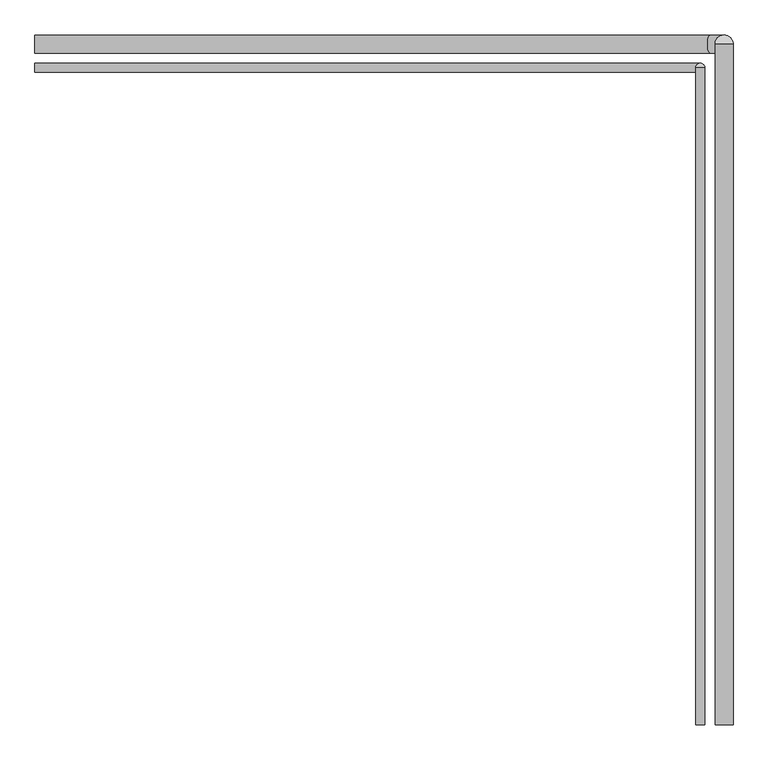
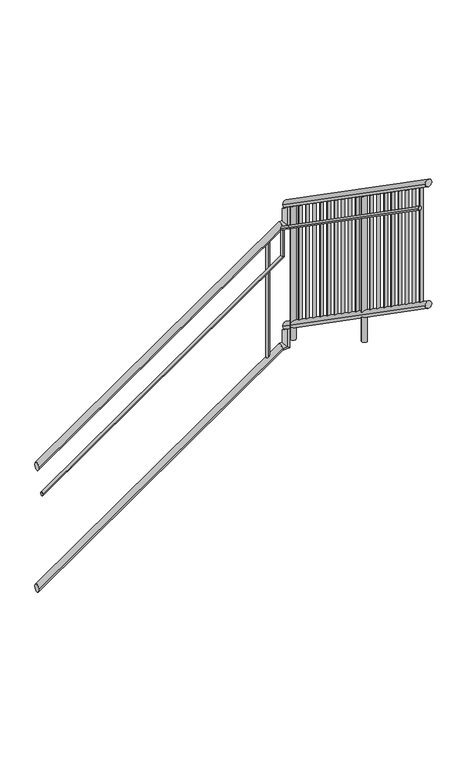
"""IFC4 building model written with IfcOpenShell, lengths in millimetres: railing geometry."""

import ifcopenshell
import ifcopenshell.guid

model = None  # the IFC model being written
_history = None  # IfcOwnerHistory: only IFC2X3 demands one
_inside = {}  # id of a spatial element -> (the spatial element, [elements in it])
_under = {}  # id of a project, library or spatial element -> (it, [spatial elements below it])
_declared = {}  # id of a project -> (the project, [libraries it declares])
_typed = {}  # id of a type object -> (the type object, [elements of that type])
_made_of = {}  # id of a material, layer set ... -> (it, [elements and type objects made of it])


def new_model(schema):
    """Start an empty IFC model of exactly this schema.

    Asked for "IFC4X3", IfcOpenShell would pick the latest addendum, in which some entities
    have other attributes; the version numbers below select the first issue.
    IFC2X3 requires an IfcOwnerHistory on every rooted entity: one is made here for all.
    """
    global model, _history
    if schema == "IFC4X3":
        model = ifcopenshell.file(schema_version=(4, 3, 0, 0))
    else:
        model = ifcopenshell.file(schema=schema)
    _inside.clear()
    _under.clear()
    _declared.clear()
    _typed.clear()
    _made_of.clear()
    _history = None
    if model.schema == "IFC2X3":
        org = make("IfcOrganization", Name="unknown")
        user = make(
            "IfcPersonAndOrganization",
            ThePerson=make("IfcPerson", FamilyName="unknown"),
            TheOrganization=org,
        )
        app = make(
            "IfcApplication",
            ApplicationDeveloper=org,
            Version="unknown",
            ApplicationFullName="unknown",
            ApplicationIdentifier="unknown",
        )
        _history = make(
            "IfcOwnerHistory",
            OwningUser=user,
            OwningApplication=app,
            ChangeAction="ADDED",
            CreationDate=0,
        )
    return model


def make(cls, **values):
    """One entity of the class cls with the attributes given. An attribute that is None is left unset."""
    return model.create_entity(
        cls, **{name: value for name, value in values.items() if value is not None}
    )


def rooted(cls, **values):
    """An entity with a GlobalId (a new one), such as an element, a storey or a relation."""
    return make(cls, GlobalId=ifcopenshell.guid.new(), OwnerHistory=_history, **values)


def si_unit(unit_type, name, prefix=None):
    """IfcSIUnit, for example si_unit("LENGTHUNIT", "METRE", prefix="MILLI")."""
    return make("IfcSIUnit", UnitType=unit_type, Prefix=prefix, Name=name)


def assignment(units):
    """IfcUnitAssignment: the units of a project."""
    return None if units is None else make("IfcUnitAssignment", Units=units)


def point(xyz):
    """IfcCartesianPoint."""
    return None if xyz is None else make("IfcCartesianPoint", Coordinates=xyz)


def direction(xyz):
    """IfcDirection."""
    return None if xyz is None else make("IfcDirection", DirectionRatios=xyz)


def frame(location, z_axis=None, x_axis=None):
    """IfcAxis2Placement3D, a coordinate frame: its origin and axes. An axis left out is left unset."""
    return make(
        "IfcAxis2Placement3D",
        Location=point(location),
        Axis=direction(z_axis),
        RefDirection=direction(x_axis),
    )


def origin():
    """The frame at (0, 0, 0) with its axes left unset."""
    return frame((0.0, 0.0, 0.0))


def place(relative_to, where):
    """IfcLocalPlacement: puts the frame where relative to a parent placement (None: the world)."""
    return make(
        "IfcLocalPlacement", PlacementRelTo=relative_to, RelativePlacement=where
    )


def context(
    kind, dimensions, precision=None, world=None, true_north=None, identifier=None
):
    """IfcGeometricRepresentationContext, for example the 3D "Model" context."""
    return make(
        "IfcGeometricRepresentationContext",
        ContextIdentifier=identifier,
        ContextType=kind,
        CoordinateSpaceDimension=dimensions,
        Precision=precision,
        WorldCoordinateSystem=world,
        TrueNorth=true_north,
    )


def project(units=None, contexts=None):
    """IfcProject with its units and contexts."""
    return rooted(
        "IfcProject",
        Name="project",
        RepresentationContexts=contexts,
        UnitsInContext=assignment(units),
    )


def spatial(cls, under=None, at=None, **own):
    """A site, building, storey or space (cls), placed at a placement, below another one or the project."""
    s = rooted(cls, ObjectPlacement=at, **own)
    if under is not None:
        _under.setdefault(under.id(), (under, []))[1].append(s)
    return s


def circle_curve(where, radius):
    """IfcCircle in the frame where."""
    return make("IfcCircle", Position=where, Radius=radius)


def ellipse_curve(where, semi_axis1, semi_axis2):
    """IfcEllipse in the frame where."""
    return make(
        "IfcEllipse", Position=where, SemiAxis1=semi_axis1, SemiAxis2=semi_axis2
    )


def shape(context_of_items, identifier, shape_type, items):
    """IfcShapeRepresentation: the items that make up one representation, for example the "Body"."""
    return make(
        "IfcShapeRepresentation",
        ContextOfItems=context_of_items,
        RepresentationIdentifier=identifier,
        RepresentationType=shape_type,
        Items=items,
    )


def source(mapping_origin, context_of_items, identifier, shape_type, items):
    """IfcRepresentationMap: a shape defined once, which mapped items show again and again."""
    return make(
        "IfcRepresentationMap",
        MappingOrigin=mapping_origin,
        MappedRepresentation=shape(context_of_items, identifier, shape_type, items),
    )


def transform(
    local_origin,
    x_axis=None,
    y_axis=None,
    z_axis=None,
    scale=None,
    scale2=None,
    scale3=None,
    uniform=True,
):
    """IfcCartesianTransformationOperator3D, or its non-uniform kind. x_axis, y_axis, z_axis: its Axis1, 2, 3."""
    if uniform:
        return make(
            "IfcCartesianTransformationOperator3D",
            Axis1=direction(x_axis),
            Axis2=direction(y_axis),
            LocalOrigin=point(local_origin),
            Scale=scale,
            Axis3=direction(z_axis),
        )
    return make(
        "IfcCartesianTransformationOperator3DnonUniform",
        Axis1=direction(x_axis),
        Axis2=direction(y_axis),
        LocalOrigin=point(local_origin),
        Scale=scale,
        Axis3=direction(z_axis),
        Scale2=scale2,
        Scale3=scale3,
    )


def mapped(mapping_source, mapping_target):
    """IfcMappedItem: shows the shape of a source again, moved by a transform."""
    return make(
        "IfcMappedItem", MappingSource=mapping_source, MappingTarget=mapping_target
    )


def made_of(thing, what):
    """Note that an element or type object is made of a material, layer set ...; save() writes the relation."""
    if what is not None:
        _made_of.setdefault(what.id(), (what, []))[1].append(thing)
    return thing


def element(
    cls,
    number,
    at=None,
    inside=None,
    cuts=None,
    type_object=None,
    material=None,
    context=None,
    identifier="Body",
    shape_type=None,
    held_by="IfcProductDefinitionShape",
    body=None,
    shapes=None,
    **own,
):
    """One element of the class cls, such as IfcWall. Its Tag is "e" and its number.

    at: its placement. inside: the storey or other place that contains it. cuts: it is an
    opening in that element (IfcRelVoidsElement). A single representation is given by context,
    identifier, shape_type and body (its items); several are given by shapes. held_by: the class
    of the entity that holds the representations. save() writes the other relations.
    """
    e = rooted(cls, Tag="e%d" % number, ObjectPlacement=at, **own)
    if body is not None:
        shapes = [shape(context, identifier, shape_type, body)]
    if shapes is not None:
        e.Representation = make(held_by, Representations=shapes)
    if inside is not None:
        _inside.setdefault(inside.id(), (inside, []))[1].append(e)
    if cuts is not None:
        rooted(
            "IfcRelVoidsElement", RelatingBuildingElement=cuts, RelatedOpeningElement=e
        )
    if type_object is not None:
        _typed.setdefault(type_object.id(), (type_object, []))[1].append(e)
    return made_of(e, material)


def aggregate(whole, parts):
    """IfcRelAggregates: a whole, such as a stair, and the parts it consists of."""
    return rooted("IfcRelAggregates", RelatingObject=whole, RelatedObjects=parts)


def save(model, path):
    """Write the relations noted so far, then the file.

    IfcRelAggregates (storeys below a building ...), IfcRelContainedInSpatialStructure (elements
    in a storey), IfcRelDefinesByType, IfcRelAssociatesMaterial and IfcRelDeclares: one each for
    every whole, place, type object, material and project.
    """
    for whole, parts in _under.values():
        aggregate(whole, parts)
    for where, things in _inside.values():
        rooted(
            "IfcRelContainedInSpatialStructure",
            RelatedElements=things,
            RelatingStructure=where,
        )
    for kind, things in _typed.values():
        rooted("IfcRelDefinesByType", RelatedObjects=things, RelatingType=kind)
    for what, things in _made_of.values():
        rooted("IfcRelAssociatesMaterial", RelatedObjects=things, RelatingMaterial=what)
    for by, libraries in _declared.values():
        rooted("IfcRelDeclares", RelatingContext=by, RelatedDefinitions=libraries)
    model.write(path)


def plane_surface(at):
    """IfcPlane: the flat surface through the origin of the frame at, square to its z axis."""
    return make("IfcPlane", Position=at)


def cylinder_surface(at, radius):
    """IfcCylindricalSurface: all points at the distance radius from the z axis of the frame at."""
    return make("IfcCylindricalSurface", Position=at, Radius=radius)


def advanced_brep(points, edges, surfaces, faces):
    """IfcAdvancedBrep: a solid bounded by faces that lie on surfaces and meet in shared edges.

    An edge is (start, end): straight between two places in points (the first is 0);
    or (start, end, curve); or (start, end, curve, False) where it runs against its curve.
    A face is (place in surfaces, loops), or (place, loops, False) where it looks against
    its surface's normal. A loop lists edges by number (the first is 1), with a minus sign
    where the edge is run from its end to its start. The first loop is the outer one.
    """
    corners = [point(p) for p in points]
    vertices = [make("IfcVertexPoint", VertexGeometry=c) for c in corners]
    made = []
    for start, end, *more in edges:
        made.append(
            make(
                "IfcEdgeCurve",
                EdgeStart=vertices[start],
                EdgeEnd=vertices[end],
                EdgeGeometry=more[0] if more else make("IfcPolyline", Points=[corners[start], corners[end]]),
                SameSense=more[1] if len(more) > 1 else True,
            )
        )
    hull = []
    for where, loops, *sense in faces:
        bounds = []
        for j, loop in enumerate(loops):
            ring = [make("IfcOrientedEdge", EdgeElement=made[abs(k) - 1], Orientation=k > 0) for k in loop]
            bounds.append(
                make(
                    "IfcFaceOuterBound" if j == 0 else "IfcFaceBound",
                    Bound=make("IfcEdgeLoop", EdgeList=ring),
                    Orientation=True,
                )
            )
        hull.append(make("IfcAdvancedFace", Bounds=bounds, FaceSurface=surfaces[where], SameSense=sense[0] if sense else True))
    return make("IfcAdvancedBrep", Outer=make("IfcClosedShell", CfsFaces=hull))


def railing_cb7ceb08(model_context):
    return source(origin(), model_context, "Body", "AdvancedBrep", [
        advanced_brep(
        [(679.725551, -1750.2965465, 1656.5760546), (679.725551, -1801.0965465, 1656.5760546), (2577.6800324, -1750.2965465, 2974.6), (2577.6800324, -1801.0965465, 2974.6), (2617.625551, -1750.2965465, 2974.6), (2617.625551, -1801.0965465, 2974.6), (2617.625551, -1750.2965465, 3090.3743314), (2617.625551, -1801.0965465, 3125.6521091)],
        [
            (0, 1, ellipse_curve(frame((679.725551, -1775.6965465, 1656.5760546), z_axis=(-1.0, 0.0, 0.0), x_axis=(0.0, 0.0, -0.9999999999999999)), 30.9239454, 25.4)),
            (1, 0, ellipse_curve(frame((679.725551, -1775.6965465, 1656.5760546), z_axis=(-1.0, 0.0, 0.0), x_axis=(0.0, 0.0, -0.9999999999999999)), 30.9239454, 25.4)),
            (0, 2),
            (2, 3, ellipse_curve(frame((2577.6800324, -1775.6965465, 2974.6), z_axis=(-0.9542981624401503, 0.0, -0.2988561814039527), x_axis=(0.2988561814039518, 0.0, -0.9542981624401508)), 26.6164193, 25.4)),
            (3, 1),
            (3, 2, ellipse_curve(frame((2577.6800324, -1775.6965465, 2974.6), z_axis=(-0.9542981624401503, 0.0, -0.2988561814039527), x_axis=(0.2988561814039518, 0.0, -0.9542981624401508)), 26.6164193, 25.4)),
            (2, 4),
            (4, 5, ellipse_curve(frame((2617.625551, -1775.6965465, 2974.6), z_axis=(-0.7071067811865474, 0.0, -0.7071067811865476), x_axis=(-0.7071067811865478, 0.0, 0.7071067811865472)), 35.9210245, 25.4)),
            (5, 3),
            (5, 4, ellipse_curve(frame((2617.625551, -1775.6965465, 2974.6), z_axis=(-0.7071067811865474, 0.0, -0.7071067811865476), x_axis=(-0.7071067811865478, 0.0, 0.7071067811865472)), 35.9210245, 25.4)),
            (6, 7, ellipse_curve(frame((2617.625551, -1775.6965465, 3108.0132202), z_axis=(0.0, 0.5703958094953442, 0.8213699656732958), x_axis=(0.0, 0.8213699656732958, -0.5703958094953442)), 30.9239454, 25.4)),
            (7, 6, ellipse_curve(frame((2617.625551, -1775.6965465, 3108.0132202), z_axis=(0.0, 0.5703958094953442, 0.8213699656732958), x_axis=(0.0, 0.8213699656732958, -0.5703958094953442)), 30.9239454, 25.4)),
            (4, 6),
            (7, 5),
        ],
        [
            plane_surface(frame((679.725551, -1775.6965465, 1687.5), z_axis=(-1.0, 0.0, 0.0), x_axis=(0.0, 1.0, 0.0))),
            cylinder_surface(frame((694.2136045, -1775.6965465, 1666.6372029), z_axis=(-0.8213699656732956, 0.0, -0.5703958094953446), x_axis=(0.0, -1.0, 0.0)), 25.4),
            cylinder_surface(frame((2569.725551, -1775.6965465, 2974.6), z_axis=(-1.0, 0.0, 0.0), x_axis=(0.0, -1.0, 0.0)), 25.4),
            plane_surface(frame((2592.225551, -1775.6965465, 3108.0132202), z_axis=(0.0, 0.5703958094953442, 0.8213699656732958), x_axis=(1.0, 0.0, 0.0))),
            cylinder_surface(frame((2617.625551, -1775.6965465, 3000.0), z_axis=(0.0, 0.0, -1.0), x_axis=(0.0, -1.0, 0.0)), 25.4),
        ],
        [
            (0, [[1, 2]]),
            (1, [[-1, 3, 4, 5]]),
            (1, [[-2, -5, 6, -3]]),
            (2, [[-4, 7, 8, 9]]),
            (2, [[-6, -9, 10, -7]]),
            (3, [[11, 12]]),
            (4, [[-8, 13, -12, 14]]),
            (4, [[-10, -14, -11, -13]]),
        ],
    ),
        advanced_brep(
        [(2643.025551, -1775.6965465, 3138.9371657), (2592.225551, -1775.6965465, 3138.9371657), (2643.025551, -3691.0965465, 4469.0760546), (2592.225551, -3691.0965465, 4469.0760546)],
        [
            (0, 1, ellipse_curve(frame((2617.625551, -1775.6965465, 3138.9371657), z_axis=(0.0, 1.0, 0.0), x_axis=(0.0, 0.0, -1.0)), 30.9239454, 25.4)),
            (1, 0, ellipse_curve(frame((2617.625551, -1775.6965465, 3138.9371657), z_axis=(0.0, 1.0, 0.0), x_axis=(0.0, 0.0, -1.0)), 30.9239454, 25.4)),
            (2, 3, ellipse_curve(frame((2617.625551, -3691.0965465, 4469.0760546), z_axis=(0.0, -1.0, 0.0), x_axis=(0.0, 0.0, -1.0)), 30.9239454, 25.4)),
            (3, 2, ellipse_curve(frame((2617.625551, -3691.0965465, 4469.0760546), z_axis=(0.0, -1.0, 0.0), x_axis=(0.0, 0.0, -1.0)), 30.9239454, 25.4)),
            (0, 2),
            (3, 1),
        ],
        [
            plane_surface(frame((2617.625551, -1775.6965465, 3169.8611111), z_axis=(0.0, 1.0, 0.0), x_axis=(0.0, 0.0, -1.0))),
            plane_surface(frame((2617.625551, -3691.0965465, 4500.0), z_axis=(0.0, -1.0, 0.0), x_axis=(0.0, 0.0, -1.0))),
            cylinder_surface(frame((2617.625551, -1790.1846001, 3148.998314), z_axis=(0.0, 0.8213699656732958, -0.5703958094953442), x_axis=(-1.0, 0.0, 0.0)), 25.4),
        ],
        [
            (0, [[1, 2]]),
            (1, [[3, 4]]),
            (2, [[-1, 5, -4, 6]]),
            (2, [[-2, -6, -3, -5]]),
        ],
    ),
        advanced_brep(
        [(679.725551, -1829.9965465, 1472.0380273), (679.725551, -1855.3965465, 1472.0380273), (2550.625551, -1829.9965465, 2771.2741384), (2550.625551, -1855.3965465, 2771.2741384), (2550.625551, -1829.9965465, 2976.645499), (2550.625551, -1855.3965465, 2994.2843879)],
        [
            (0, 1, ellipse_curve(frame((679.725551, -1842.6965465, 1472.0380273), z_axis=(-1.0, 0.0, 0.0), x_axis=(0.0, 0.0, -1.0)), 15.4619727, 12.7)),
            (1, 0, ellipse_curve(frame((679.725551, -1842.6965465, 1472.0380273), z_axis=(-1.0, 0.0, 0.0), x_axis=(0.0, 0.0, -1.0)), 15.4619727, 12.7)),
            (0, 2),
            (2, 3, ellipse_curve(frame((2550.625551, -1842.6965465, 2771.2741384), z_axis=(-0.4634674694650399, 0.0, -0.8861139344055438), x_axis=(-0.8861139344055436, 0.0, 0.46346746946504)), 14.3322427, 12.7)),
            (3, 1),
            (3, 2, ellipse_curve(frame((2550.625551, -1842.6965465, 2771.2741384), z_axis=(-0.4634674694650399, 0.0, -0.8861139344055438), x_axis=(-0.8861139344055436, 0.0, 0.46346746946504)), 14.3322427, 12.7)),
            (4, 5, ellipse_curve(frame((2550.625551, -1842.6965465, 2985.4649435), z_axis=(0.0, 0.5703958094953442, 0.8213699656732959), x_axis=(0.0, 0.821369965673296, -0.5703958094953439)), 15.4619727, 12.7)),
            (5, 4, ellipse_curve(frame((2550.625551, -1842.6965465, 2985.4649435), z_axis=(0.0, 0.5703958094953442, 0.8213699656732959), x_axis=(0.0, 0.821369965673296, -0.5703958094953439)), 15.4619727, 12.7)),
            (2, 4),
            (5, 3),
        ],
        [
            plane_surface(frame((679.725551, -1842.6965465, 1487.5), z_axis=(-1.0, 0.0, 0.0), x_axis=(0.0, 1.0, 0.0))),
            cylinder_surface(frame((686.9695777, -1842.6965465, 1477.0686014), z_axis=(-0.8213699656732956, 0.0, -0.5703958094953444), x_axis=(0.0, -1.0, 0.0)), 12.7),
            plane_surface(frame((2537.925551, -1842.6965465, 2985.4649435), z_axis=(0.0, 0.5703958094953442, 0.8213699656732959), x_axis=(1.0, 0.0, 0.0))),
            cylinder_surface(frame((2550.625551, -1842.6965465, 2777.9166667), z_axis=(0.0, 0.0, -1.0), x_axis=(0.0, -1.0, 0.0)), 12.7),
        ],
        [
            (0, [[1, 2]]),
            (1, [[-1, 3, 4, 5]]),
            (1, [[-2, -5, 6, -3]]),
            (2, [[7, 8]]),
            (3, [[-4, 9, -8, 10]]),
            (3, [[-6, -10, -7, -9]]),
        ],
    ),
        advanced_brep(
        [(2563.325551, -1842.6965465, 3000.9269162), (2537.925551, -1842.6965465, 3000.9269162), (2563.325551, -3691.0965465, 4284.5380273), (2537.925551, -3691.0965465, 4284.5380273)],
        [
            (0, 1, ellipse_curve(frame((2550.625551, -1842.6965465, 3000.9269162), z_axis=(0.0, 1.0, 0.0), x_axis=(0.0, 0.0, -1.0)), 15.4619727, 12.7)),
            (1, 0, ellipse_curve(frame((2550.625551, -1842.6965465, 3000.9269162), z_axis=(0.0, 1.0, 0.0), x_axis=(0.0, 0.0, -1.0)), 15.4619727, 12.7)),
            (2, 3, ellipse_curve(frame((2550.625551, -3691.0965465, 4284.5380273), z_axis=(0.0, -1.0, 0.0), x_axis=(0.0, 0.0, -1.0)), 15.4619727, 12.7)),
            (3, 2, ellipse_curve(frame((2550.625551, -3691.0965465, 4284.5380273), z_axis=(0.0, -1.0, 0.0), x_axis=(0.0, 0.0, -1.0)), 15.4619727, 12.7)),
            (0, 2),
            (3, 1),
        ],
        [
            plane_surface(frame((2550.625551, -1842.6965465, 3016.3888889), z_axis=(0.0, 1.0, 0.0), x_axis=(0.0, 0.0, -1.0))),
            plane_surface(frame((2550.625551, -3691.0965465, 4300.0), z_axis=(0.0, -1.0, 0.0), x_axis=(0.0, 0.0, -1.0))),
            cylinder_surface(frame((2550.625551, -1849.9405733, 3005.9574903), z_axis=(0.0, 0.8213699656732959, -0.5703958094953442), x_axis=(-1.0, 0.0, 0.0)), 12.7),
        ],
        [
            (0, [[1, 2]]),
            (1, [[3, 4]]),
            (2, [[-1, 5, -4, 6]]),
            (2, [[-2, -6, -3, -5]]),
        ],
    ),
        advanced_brep(
        [(679.725551, -1750.2965465, 656.5760546), (679.725551, -1801.0965465, 656.5760546), (2577.6800324, -1750.2965465, 1974.6), (2577.6800324, -1801.0965465, 1974.6), (2617.625551, -1750.2965465, 1974.6), (2617.625551, -1801.0965465, 1974.6), (2617.625551, -1750.2965465, 2090.3743314), (2617.625551, -1801.0965465, 2125.6521091)],
        [
            (0, 1, ellipse_curve(frame((679.725551, -1775.6965465, 656.5760546), z_axis=(-1.0, 0.0, 0.0), x_axis=(0.0, 0.0, -1.0)), 30.9239454, 25.4)),
            (1, 0, ellipse_curve(frame((679.725551, -1775.6965465, 656.5760546), z_axis=(-1.0, 0.0, 0.0), x_axis=(0.0, 0.0, -1.0)), 30.9239454, 25.4)),
            (0, 2),
            (2, 3, ellipse_curve(frame((2577.6800324, -1775.6965465, 1974.6), z_axis=(-0.9542981624401505, 0.0, -0.29885618140395265), x_axis=(0.2988561814039529, 0.0, -0.9542981624401503)), 26.6164193, 25.4)),
            (3, 1),
            (3, 2, ellipse_curve(frame((2577.6800324, -1775.6965465, 1974.6), z_axis=(-0.9542981624401505, 0.0, -0.29885618140395265), x_axis=(0.2988561814039529, 0.0, -0.9542981624401503)), 26.6164193, 25.4)),
            (2, 4),
            (4, 5, ellipse_curve(frame((2617.625551, -1775.6965465, 1974.6), z_axis=(-0.7071067811865475, 0.0, -0.7071067811865475), x_axis=(-0.7071067811865476, 0.0, 0.7071067811865474)), 35.9210245, 25.4)),
            (5, 3),
            (5, 4, ellipse_curve(frame((2617.625551, -1775.6965465, 1974.6), z_axis=(-0.7071067811865475, 0.0, -0.7071067811865475), x_axis=(-0.7071067811865476, 0.0, 0.7071067811865474)), 35.9210245, 25.4)),
            (6, 7, ellipse_curve(frame((2617.625551, -1775.6965465, 2108.0132202), z_axis=(0.0, 0.5703958094953442, 0.8213699656732958), x_axis=(0.0, 0.8213699656732958, -0.5703958094953442)), 30.9239454, 25.4)),
            (7, 6, ellipse_curve(frame((2617.625551, -1775.6965465, 2108.0132202), z_axis=(0.0, 0.5703958094953442, 0.8213699656732958), x_axis=(0.0, 0.8213699656732958, -0.5703958094953442)), 30.9239454, 25.4)),
            (4, 6),
            (7, 5),
        ],
        [
            plane_surface(frame((679.725551, -1775.6965465, 687.5), z_axis=(-1.0, 0.0, 0.0), x_axis=(0.0, 1.0, 0.0))),
            cylinder_surface(frame((694.2136045, -1775.6965465, 666.6372029), z_axis=(-0.8213699656732956, 0.0, -0.5703958094953445), x_axis=(0.0, -1.0, 0.0)), 25.4),
            cylinder_surface(frame((2569.725551, -1775.6965465, 1974.6), z_axis=(-1.0, 0.0, 0.0), x_axis=(0.0, -1.0, 0.0)), 25.4),
            plane_surface(frame((2592.225551, -1775.6965465, 2108.0132202), z_axis=(0.0, 0.5703958094953442, 0.8213699656732958), x_axis=(1.0, 0.0, 0.0))),
            cylinder_surface(frame((2617.625551, -1775.6965465, 2000.0), z_axis=(0.0, 0.0, -1.0), x_axis=(0.0, -1.0, 0.0)), 25.4),
        ],
        [
            (0, [[1, 2]]),
            (1, [[-1, 3, 4, 5]]),
            (1, [[-2, -5, 6, -3]]),
            (2, [[-4, 7, 8, 9]]),
            (2, [[-6, -9, 10, -7]]),
            (3, [[11, 12]]),
            (4, [[-8, 13, -12, 14]]),
            (4, [[-10, -14, -11, -13]]),
        ],
    ),
        advanced_brep(
        [(2643.025551, -1775.6965465, 2138.9371657), (2592.225551, -1775.6965465, 2138.9371657), (2643.025551, -3691.0965465, 3469.0760546), (2592.225551, -3691.0965465, 3469.0760546)],
        [
            (0, 1, ellipse_curve(frame((2617.625551, -1775.6965465, 2138.9371657), z_axis=(0.0, 1.0, 0.0), x_axis=(0.0, 0.0, -1.0)), 30.9239454, 25.4)),
            (1, 0, ellipse_curve(frame((2617.625551, -1775.6965465, 2138.9371657), z_axis=(0.0, 1.0, 0.0), x_axis=(0.0, 0.0, -1.0)), 30.9239454, 25.4)),
            (2, 3, ellipse_curve(frame((2617.625551, -3691.0965465, 3469.0760546), z_axis=(0.0, -1.0, 0.0), x_axis=(0.0, 0.0, -1.0)), 30.9239454, 25.4)),
            (3, 2, ellipse_curve(frame((2617.625551, -3691.0965465, 3469.0760546), z_axis=(0.0, -1.0, 0.0), x_axis=(0.0, 0.0, -1.0)), 30.9239454, 25.4)),
            (0, 2),
            (3, 1),
        ],
        [
            plane_surface(frame((2617.625551, -1775.6965465, 2169.8611111), z_axis=(0.0, 1.0, 0.0), x_axis=(0.0, 0.0, -1.0))),
            plane_surface(frame((2617.625551, -3691.0965465, 3500.0), z_axis=(0.0, -1.0, 0.0), x_axis=(0.0, 0.0, -1.0))),
            cylinder_surface(frame((2617.625551, -1790.1846001, 2148.998314), z_axis=(0.0, 0.8213699656732958, -0.5703958094953442), x_axis=(-1.0, 0.0, 0.0)), 25.4),
        ],
        [
            (0, [[1, 2]]),
            (1, [[3, 4]]),
            (2, [[-1, 5, -4, 6]]),
            (2, [[-2, -6, -3, -5]]),
        ],
    ),
        advanced_brep(
        [(2605.125551, -3595.3265465, 4371.6451647), (2605.125551, -3595.3265465, 3433.4930556), (2630.125551, -3595.3265465, 3433.4930556), (2630.125551, -3595.3265465, 4371.6451647)],
        [
            (0, 1),
            (1, 2, ellipse_curve(frame((2617.625551, -3595.3265465, 3433.4930556), z_axis=(0.0, 0.5703958094953444, 0.8213699656732956), x_axis=(0.0, -0.8213699656732956, 0.5703958094953445)), 15.2184771, 12.5)),
            (2, 3),
            (3, 0, ellipse_curve(frame((2617.625551, -3595.3265465, 4371.6451647), z_axis=(0.0, -0.5703958094953457, -0.8213699656732947), x_axis=(0.0, -0.8213699656732947, 0.5703958094953456)), 15.2184771, 12.5)),
            (0, 3, ellipse_curve(frame((2617.625551, -3595.3265465, 4371.6451647), z_axis=(0.0, -0.5703958094953457, -0.8213699656732947), x_axis=(0.0, -0.8213699656732947, 0.5703958094953456)), 15.2184771, 12.5)),
            (2, 1, ellipse_curve(frame((2617.625551, -3595.3265465, 3433.4930556), z_axis=(0.0, 0.5703958094953444, 0.8213699656732956), x_axis=(0.0, -0.8213699656732956, 0.5703958094953445)), 15.2184771, 12.5)),
        ],
        [
            cylinder_surface(frame((2617.625551, -3595.3265465, 3333.4930556), z_axis=(0.0, 0.0, 1.0), x_axis=(1.0, 0.0, 0.0)), 12.5),
            plane_surface(frame((2642.625551, -3620.3265465, 4389.0062758), z_axis=(0.0, 0.5703958094953457, 0.8213699656732947), x_axis=(-1.0, 0.0, 0.0))),
            plane_surface(frame((2642.625551, -3570.3265465, 3416.1319444), z_axis=(0.0, -0.5703958094953444, -0.8213699656732956), x_axis=(-1.0, 0.0, 0.0))),
        ],
        [
            (0, [[1, 2, 3, 4]]),
            (0, [[-1, 5, -3, 6]]),
            (1, [[-4, -5]]),
            (2, [[-2, -6]]),
        ],
    ),
        advanced_brep(
        [(2605.125551, -3499.5565465, 4305.1382202), (2605.125551, -3499.5565465, 3366.9861111), (2630.125551, -3499.5565465, 3366.9861111), (2630.125551, -3499.5565465, 4305.1382202)],
        [
            (0, 1),
            (1, 2, ellipse_curve(frame((2617.625551, -3499.5565465, 3366.9861111), z_axis=(0.0, 0.5703958094953444, 0.8213699656732956), x_axis=(0.0, -0.8213699656732956, 0.5703958094953445)), 15.2184771, 12.5)),
            (2, 3),
            (3, 0, ellipse_curve(frame((2617.625551, -3499.5565465, 4305.1382202), z_axis=(0.0, -0.5703958094953457, -0.8213699656732947), x_axis=(0.0, -0.8213699656732947, 0.5703958094953456)), 15.2184771, 12.5)),
            (0, 3, ellipse_curve(frame((2617.625551, -3499.5565465, 4305.1382202), z_axis=(0.0, -0.5703958094953457, -0.8213699656732947), x_axis=(0.0, -0.8213699656732947, 0.5703958094953456)), 15.2184771, 12.5)),
            (2, 1, ellipse_curve(frame((2617.625551, -3499.5565465, 3366.9861111), z_axis=(0.0, 0.5703958094953444, 0.8213699656732956), x_axis=(0.0, -0.8213699656732956, 0.5703958094953445)), 15.2184771, 12.5)),
        ],
        [
            cylinder_surface(frame((2617.625551, -3499.5565465, 3266.9861111), z_axis=(0.0, 0.0, 1.0), x_axis=(1.0, 0.0, 0.0)), 12.5),
            plane_surface(frame((2642.625551, -3524.5565465, 4322.4993314), z_axis=(0.0, 0.5703958094953457, 0.8213699656732947), x_axis=(-1.0, 0.0, 0.0))),
            plane_surface(frame((2642.625551, -3474.5565465, 3349.625), z_axis=(0.0, -0.5703958094953444, -0.8213699656732956), x_axis=(-1.0, 0.0, 0.0))),
        ],
        [
            (0, [[1, 2, 3, 4]]),
            (0, [[-1, 5, -3, 6]]),
            (1, [[-4, -5]]),
            (2, [[-2, -6]]),
        ],
    ),
        advanced_brep(
        [(2605.125551, -3403.7865465, 4238.6312758), (2605.125551, -3403.7865465, 3300.4791667), (2630.125551, -3403.7865465, 3300.4791667), (2630.125551, -3403.7865465, 4238.6312758)],
        [
            (0, 1),
            (1, 2, ellipse_curve(frame((2617.625551, -3403.7865465, 3300.4791667), z_axis=(0.0, 0.5703958094953444, 0.8213699656732956), x_axis=(0.0, -0.8213699656732956, 0.5703958094953445)), 15.2184771, 12.5)),
            (2, 3),
            (3, 0, ellipse_curve(frame((2617.625551, -3403.7865465, 4238.6312758), z_axis=(0.0, -0.5703958094953457, -0.8213699656732947), x_axis=(0.0, -0.8213699656732947, 0.5703958094953456)), 15.2184771, 12.5)),
            (0, 3, ellipse_curve(frame((2617.625551, -3403.7865465, 4238.6312758), z_axis=(0.0, -0.5703958094953457, -0.8213699656732947), x_axis=(0.0, -0.8213699656732947, 0.5703958094953456)), 15.2184771, 12.5)),
            (2, 1, ellipse_curve(frame((2617.625551, -3403.7865465, 3300.4791667), z_axis=(0.0, 0.5703958094953444, 0.8213699656732956), x_axis=(0.0, -0.8213699656732956, 0.5703958094953445)), 15.2184771, 12.5)),
        ],
        [
            cylinder_surface(frame((2617.625551, -3403.7865465, 3200.4791667), z_axis=(0.0, 0.0, 1.0), x_axis=(1.0, 0.0, 0.0)), 12.5),
            plane_surface(frame((2642.625551, -3428.7865465, 4255.9923869), z_axis=(0.0, 0.5703958094953457, 0.8213699656732947), x_axis=(-1.0, 0.0, 0.0))),
            plane_surface(frame((2642.625551, -3378.7865465, 3283.1180556), z_axis=(0.0, -0.5703958094953444, -0.8213699656732956), x_axis=(-1.0, 0.0, 0.0))),
        ],
        [
            (0, [[1, 2, 3, 4]]),
            (0, [[-1, 5, -3, 6]]),
            (1, [[-4, -5]]),
            (2, [[-2, -6]]),
        ],
    ),
        advanced_brep(
        [(2605.125551, -3308.0165465, 4172.1243314), (2605.125551, -3308.0165465, 3233.9722222), (2630.125551, -3308.0165465, 3233.9722222), (2630.125551, -3308.0165465, 4172.1243314)],
        [
            (0, 1),
            (1, 2, ellipse_curve(frame((2617.625551, -3308.0165465, 3233.9722222), z_axis=(0.0, 0.5703958094953444, 0.8213699656732956), x_axis=(0.0, -0.8213699656732956, 0.5703958094953445)), 15.2184771, 12.5)),
            (2, 3),
            (3, 0, ellipse_curve(frame((2617.625551, -3308.0165465, 4172.1243314), z_axis=(0.0, -0.5703958094953457, -0.8213699656732947), x_axis=(0.0, -0.8213699656732947, 0.5703958094953456)), 15.2184771, 12.5)),
            (0, 3, ellipse_curve(frame((2617.625551, -3308.0165465, 4172.1243314), z_axis=(0.0, -0.5703958094953457, -0.8213699656732947), x_axis=(0.0, -0.8213699656732947, 0.5703958094953456)), 15.2184771, 12.5)),
            (2, 1, ellipse_curve(frame((2617.625551, -3308.0165465, 3233.9722222), z_axis=(0.0, 0.5703958094953444, 0.8213699656732956), x_axis=(0.0, -0.8213699656732956, 0.5703958094953445)), 15.2184771, 12.5)),
        ],
        [
            cylinder_surface(frame((2617.625551, -3308.0165465, 3133.9722222), z_axis=(0.0, 0.0, 1.0), x_axis=(1.0, 0.0, 0.0)), 12.5),
            plane_surface(frame((2642.625551, -3333.0165465, 4189.4854425), z_axis=(0.0, 0.5703958094953457, 0.8213699656732947), x_axis=(-1.0, 0.0, 0.0))),
            plane_surface(frame((2642.625551, -3283.0165465, 3216.6111111), z_axis=(0.0, -0.5703958094953444, -0.8213699656732956), x_axis=(-1.0, 0.0, 0.0))),
        ],
        [
            (0, [[1, 2, 3, 4]]),
            (0, [[-1, 5, -3, 6]]),
            (1, [[-4, -5]]),
            (2, [[-2, -6]]),
        ],
    ),
        advanced_brep(
        [(2605.125551, -3212.2465465, 4105.6173869), (2605.125551, -3212.2465465, 3167.4652778), (2630.125551, -3212.2465465, 3167.4652778), (2630.125551, -3212.2465465, 4105.6173869)],
        [
            (0, 1),
            (1, 2, ellipse_curve(frame((2617.625551, -3212.2465465, 3167.4652778), z_axis=(0.0, 0.5703958094953444, 0.8213699656732956), x_axis=(0.0, -0.8213699656732956, 0.5703958094953445)), 15.2184771, 12.5)),
            (2, 3),
            (3, 0, ellipse_curve(frame((2617.625551, -3212.2465465, 4105.6173869), z_axis=(0.0, -0.5703958094953457, -0.8213699656732947), x_axis=(0.0, -0.8213699656732947, 0.5703958094953456)), 15.2184771, 12.5)),
            (0, 3, ellipse_curve(frame((2617.625551, -3212.2465465, 4105.6173869), z_axis=(0.0, -0.5703958094953457, -0.8213699656732947), x_axis=(0.0, -0.8213699656732947, 0.5703958094953456)), 15.2184771, 12.5)),
            (2, 1, ellipse_curve(frame((2617.625551, -3212.2465465, 3167.4652778), z_axis=(0.0, 0.5703958094953444, 0.8213699656732956), x_axis=(0.0, -0.8213699656732956, 0.5703958094953445)), 15.2184771, 12.5)),
        ],
        [
            cylinder_surface(frame((2617.625551, -3212.2465465, 3067.4652778), z_axis=(0.0, 0.0, 1.0), x_axis=(1.0, 0.0, 0.0)), 12.5),
            plane_surface(frame((2642.625551, -3237.2465465, 4122.978498), z_axis=(0.0, 0.5703958094953457, 0.8213699656732947), x_axis=(-1.0, 0.0, 0.0))),
            plane_surface(frame((2642.625551, -3187.2465465, 3150.1041667), z_axis=(0.0, -0.5703958094953444, -0.8213699656732956), x_axis=(-1.0, 0.0, 0.0))),
        ],
        [
            (0, [[1, 2, 3, 4]]),
            (0, [[-1, 5, -3, 6]]),
            (1, [[-4, -5]]),
            (2, [[-2, -6]]),
        ],
    ),
        advanced_brep(
        [(2605.125551, -3116.4765465, 4039.1104425), (2605.125551, -3116.4765465, 3100.9583333), (2630.125551, -3116.4765465, 3100.9583333), (2630.125551, -3116.4765465, 4039.1104425)],
        [
            (0, 1),
            (1, 2, ellipse_curve(frame((2617.625551, -3116.4765465, 3100.9583333), z_axis=(0.0, 0.5703958094953444, 0.8213699656732956), x_axis=(0.0, -0.8213699656732956, 0.5703958094953445)), 15.2184771, 12.5)),
            (2, 3),
            (3, 0, ellipse_curve(frame((2617.625551, -3116.4765465, 4039.1104425), z_axis=(0.0, -0.5703958094953457, -0.8213699656732947), x_axis=(0.0, -0.8213699656732947, 0.5703958094953456)), 15.2184771, 12.5)),
            (0, 3, ellipse_curve(frame((2617.625551, -3116.4765465, 4039.1104425), z_axis=(0.0, -0.5703958094953457, -0.8213699656732947), x_axis=(0.0, -0.8213699656732947, 0.5703958094953456)), 15.2184771, 12.5)),
            (2, 1, ellipse_curve(frame((2617.625551, -3116.4765465, 3100.9583333), z_axis=(0.0, 0.5703958094953444, 0.8213699656732956), x_axis=(0.0, -0.8213699656732956, 0.5703958094953445)), 15.2184771, 12.5)),
        ],
        [
            cylinder_surface(frame((2617.625551, -3116.4765465, 3000.9583333), z_axis=(0.0, 0.0, 1.0), x_axis=(1.0, 0.0, 0.0)), 12.5),
            plane_surface(frame((2642.625551, -3141.4765465, 4056.4715536), z_axis=(0.0, 0.5703958094953457, 0.8213699656732947), x_axis=(-1.0, 0.0, 0.0))),
            plane_surface(frame((2642.625551, -3091.4765465, 3083.5972222), z_axis=(0.0, -0.5703958094953444, -0.8213699656732956), x_axis=(-1.0, 0.0, 0.0))),
        ],
        [
            (0, [[1, 2, 3, 4]]),
            (0, [[-1, 5, -3, 6]]),
            (1, [[-4, -5]]),
            (2, [[-2, -6]]),
        ],
    ),
        advanced_brep(
        [(2605.125551, -3020.7065465, 3972.603498), (2605.125551, -3020.7065465, 3034.4513889), (2630.125551, -3020.7065465, 3034.4513889), (2630.125551, -3020.7065465, 3972.603498)],
        [
            (0, 1),
            (1, 2, ellipse_curve(frame((2617.625551, -3020.7065465, 3034.4513889), z_axis=(0.0, 0.5703958094953444, 0.8213699656732956), x_axis=(0.0, -0.8213699656732956, 0.5703958094953445)), 15.2184771, 12.5)),
            (2, 3),
            (3, 0, ellipse_curve(frame((2617.625551, -3020.7065465, 3972.603498), z_axis=(0.0, -0.5703958094953457, -0.8213699656732947), x_axis=(0.0, -0.8213699656732947, 0.5703958094953456)), 15.2184771, 12.5)),
            (0, 3, ellipse_curve(frame((2617.625551, -3020.7065465, 3972.603498), z_axis=(0.0, -0.5703958094953457, -0.8213699656732947), x_axis=(0.0, -0.8213699656732947, 0.5703958094953456)), 15.2184771, 12.5)),
            (2, 1, ellipse_curve(frame((2617.625551, -3020.7065465, 3034.4513889), z_axis=(0.0, 0.5703958094953444, 0.8213699656732956), x_axis=(0.0, -0.8213699656732956, 0.5703958094953445)), 15.2184771, 12.5)),
        ],
        [
            cylinder_surface(frame((2617.625551, -3020.7065465, 2934.4513889), z_axis=(0.0, 0.0, 1.0), x_axis=(1.0, 0.0, 0.0)), 12.5),
            plane_surface(frame((2642.625551, -3045.7065465, 3989.9646091), z_axis=(0.0, 0.5703958094953457, 0.8213699656732947), x_axis=(-1.0, 0.0, 0.0))),
            plane_surface(frame((2642.625551, -2995.7065465, 3017.0902778), z_axis=(0.0, -0.5703958094953444, -0.8213699656732956), x_axis=(-1.0, 0.0, 0.0))),
        ],
        [
            (0, [[1, 2, 3, 4]]),
            (0, [[-1, 5, -3, 6]]),
            (1, [[-4, -5]]),
            (2, [[-2, -6]]),
        ],
    ),
        advanced_brep(
        [(2605.125551, -2924.9365465, 3906.0965536), (2605.125551, -2924.9365465, 2967.9444444), (2630.125551, -2924.9365465, 2967.9444444), (2630.125551, -2924.9365465, 3906.0965536)],
        [
            (0, 1),
            (1, 2, ellipse_curve(frame((2617.625551, -2924.9365465, 2967.9444444), z_axis=(0.0, 0.5703958094953444, 0.8213699656732956), x_axis=(0.0, -0.8213699656732956, 0.5703958094953445)), 15.2184771, 12.5)),
            (2, 3),
            (3, 0, ellipse_curve(frame((2617.625551, -2924.9365465, 3906.0965536), z_axis=(0.0, -0.5703958094953457, -0.8213699656732947), x_axis=(0.0, -0.8213699656732947, 0.5703958094953456)), 15.2184771, 12.5)),
            (0, 3, ellipse_curve(frame((2617.625551, -2924.9365465, 3906.0965536), z_axis=(0.0, -0.5703958094953457, -0.8213699656732947), x_axis=(0.0, -0.8213699656732947, 0.5703958094953456)), 15.2184771, 12.5)),
            (2, 1, ellipse_curve(frame((2617.625551, -2924.9365465, 2967.9444444), z_axis=(0.0, 0.5703958094953444, 0.8213699656732956), x_axis=(0.0, -0.8213699656732956, 0.5703958094953445)), 15.2184771, 12.5)),
        ],
        [
            cylinder_surface(frame((2617.625551, -2924.9365465, 2867.9444444), z_axis=(0.0, 0.0, 1.0), x_axis=(1.0, 0.0, 0.0)), 12.5),
            plane_surface(frame((2642.625551, -2949.9365465, 3923.4576647), z_axis=(0.0, 0.5703958094953457, 0.8213699656732947), x_axis=(-1.0, 0.0, 0.0))),
            plane_surface(frame((2642.625551, -2899.9365465, 2950.5833333), z_axis=(0.0, -0.5703958094953444, -0.8213699656732956), x_axis=(-1.0, 0.0, 0.0))),
        ],
        [
            (0, [[1, 2, 3, 4]]),
            (0, [[-1, 5, -3, 6]]),
            (1, [[-4, -5]]),
            (2, [[-2, -6]]),
        ],
    ),
        advanced_brep(
        [(2596.625551, -2829.1665465, 3839.5896091), (2596.625551, -2829.1665465, 2650.0), (2638.625551, -2829.1665465, 2650.0), (2638.625551, -2829.1665465, 3839.5896091)],
        [
            (0, 1),
            (1, 2, circle_curve(frame((2617.625551, -2829.1665465, 2650.0), z_axis=(0.0, 0.0, 1.0), x_axis=(1.0, 0.0, 0.0)), 21.0)),
            (2, 3),
            (3, 0, ellipse_curve(frame((2617.625551, -2829.1665465, 3839.5896091), z_axis=(0.0, -0.5703958094953442, -0.8213699656732958), x_axis=(0.0, -0.8213699656732958, 0.5703958094953442)), 25.5670415, 21.0)),
            (0, 3, ellipse_curve(frame((2617.625551, -2829.1665465, 3839.5896091), z_axis=(0.0, -0.5703958094953442, -0.8213699656732958), x_axis=(0.0, -0.8213699656732958, 0.5703958094953442)), 25.5670415, 21.0)),
            (2, 1, circle_curve(frame((2617.625551, -2829.1665465, 2650.0), z_axis=(0.0, 0.0, 1.0), x_axis=(1.0, 0.0, 0.0)), 21.0)),
        ],
        [
            cylinder_surface(frame((2617.625551, -2829.1665465, 2550.0), z_axis=(0.0, 0.0, 1.0), x_axis=(1.0, 0.0, 0.0)), 21.0),
            plane_surface(frame((2659.625551, -2871.1665465, 3868.7562758), z_axis=(0.0, 0.5703958094953442, 0.8213699656732958), x_axis=(-1.0, 0.0, 0.0))),
            plane_surface(frame((2659.625551, -2787.1665465, 2650.0), z_axis=(0.0, 0.0, -1.0), x_axis=(-1.0, 0.0, 0.0))),
        ],
        [
            (0, [[1, 2, 3, 4]]),
            (0, [[-1, 5, -3, 6]]),
            (1, [[-4, -5]]),
            (2, [[-2, -6]]),
        ],
    ),
        advanced_brep(
        [(2605.125551, -2733.3965465, 3773.0826647), (2605.125551, -2733.3965465, 2834.9305556), (2630.125551, -2733.3965465, 2834.9305556), (2630.125551, -2733.3965465, 3773.0826647)],
        [
            (0, 1),
            (1, 2, ellipse_curve(frame((2617.625551, -2733.3965465, 2834.9305556), z_axis=(0.0, 0.5703958094953444, 0.8213699656732956), x_axis=(0.0, -0.8213699656732956, 0.5703958094953445)), 15.2184771, 12.5)),
            (2, 3),
            (3, 0, ellipse_curve(frame((2617.625551, -2733.3965465, 3773.0826647), z_axis=(0.0, -0.5703958094953457, -0.8213699656732947), x_axis=(0.0, -0.8213699656732947, 0.5703958094953456)), 15.2184771, 12.5)),
            (0, 3, ellipse_curve(frame((2617.625551, -2733.3965465, 3773.0826647), z_axis=(0.0, -0.5703958094953457, -0.8213699656732947), x_axis=(0.0, -0.8213699656732947, 0.5703958094953456)), 15.2184771, 12.5)),
            (2, 1, ellipse_curve(frame((2617.625551, -2733.3965465, 2834.9305556), z_axis=(0.0, 0.5703958094953444, 0.8213699656732956), x_axis=(0.0, -0.8213699656732956, 0.5703958094953445)), 15.2184771, 12.5)),
        ],
        [
            cylinder_surface(frame((2617.625551, -2733.3965465, 2734.9305556), z_axis=(0.0, 0.0, 1.0), x_axis=(1.0, 0.0, 0.0)), 12.5),
            plane_surface(frame((2642.625551, -2758.3965465, 3790.4437758), z_axis=(0.0, 0.5703958094953457, 0.8213699656732947), x_axis=(-1.0, 0.0, 0.0))),
            plane_surface(frame((2642.625551, -2708.3965465, 2817.5694444), z_axis=(0.0, -0.5703958094953444, -0.8213699656732956), x_axis=(-1.0, 0.0, 0.0))),
        ],
        [
            (0, [[1, 2, 3, 4]]),
            (0, [[-1, 5, -3, 6]]),
            (1, [[-4, -5]]),
            (2, [[-2, -6]]),
        ],
    ),
        advanced_brep(
        [(2605.125551, -2637.6265465, 3706.5757202), (2605.125551, -2637.6265465, 2768.4236111), (2630.125551, -2637.6265465, 2768.4236111), (2630.125551, -2637.6265465, 3706.5757202)],
        [
            (0, 1),
            (1, 2, ellipse_curve(frame((2617.625551, -2637.6265465, 2768.4236111), z_axis=(0.0, 0.5703958094953444, 0.8213699656732956), x_axis=(0.0, -0.8213699656732956, 0.5703958094953445)), 15.2184771, 12.5)),
            (2, 3),
            (3, 0, ellipse_curve(frame((2617.625551, -2637.6265465, 3706.5757202), z_axis=(0.0, -0.5703958094953457, -0.8213699656732947), x_axis=(0.0, -0.8213699656732947, 0.5703958094953456)), 15.2184771, 12.5)),
            (0, 3, ellipse_curve(frame((2617.625551, -2637.6265465, 3706.5757202), z_axis=(0.0, -0.5703958094953457, -0.8213699656732947), x_axis=(0.0, -0.8213699656732947, 0.5703958094953456)), 15.2184771, 12.5)),
            (2, 1, ellipse_curve(frame((2617.625551, -2637.6265465, 2768.4236111), z_axis=(0.0, 0.5703958094953444, 0.8213699656732956), x_axis=(0.0, -0.8213699656732956, 0.5703958094953445)), 15.2184771, 12.5)),
        ],
        [
            cylinder_surface(frame((2617.625551, -2637.6265465, 2668.4236111), z_axis=(0.0, 0.0, 1.0), x_axis=(1.0, 0.0, 0.0)), 12.5),
            plane_surface(frame((2642.625551, -2662.6265465, 3723.9368314), z_axis=(0.0, 0.5703958094953457, 0.8213699656732947), x_axis=(-1.0, 0.0, 0.0))),
            plane_surface(frame((2642.625551, -2612.6265465, 2751.0625), z_axis=(0.0, -0.5703958094953444, -0.8213699656732956), x_axis=(-1.0, 0.0, 0.0))),
        ],
        [
            (0, [[1, 2, 3, 4]]),
            (0, [[-1, 5, -3, 6]]),
            (1, [[-4, -5]]),
            (2, [[-2, -6]]),
        ],
    ),
        advanced_brep(
        [(2605.125551, -2541.8565465, 3640.0687758), (2605.125551, -2541.8565465, 2701.9166667), (2630.125551, -2541.8565465, 2701.9166667), (2630.125551, -2541.8565465, 3640.0687758)],
        [
            (0, 1),
            (1, 2, ellipse_curve(frame((2617.625551, -2541.8565465, 2701.9166667), z_axis=(0.0, 0.5703958094953444, 0.8213699656732956), x_axis=(0.0, -0.8213699656732956, 0.5703958094953445)), 15.2184771, 12.5)),
            (2, 3),
            (3, 0, ellipse_curve(frame((2617.625551, -2541.8565465, 3640.0687758), z_axis=(0.0, -0.5703958094953457, -0.8213699656732947), x_axis=(0.0, -0.8213699656732947, 0.5703958094953456)), 15.2184771, 12.5)),
            (0, 3, ellipse_curve(frame((2617.625551, -2541.8565465, 3640.0687758), z_axis=(0.0, -0.5703958094953457, -0.8213699656732947), x_axis=(0.0, -0.8213699656732947, 0.5703958094953456)), 15.2184771, 12.5)),
            (2, 1, ellipse_curve(frame((2617.625551, -2541.8565465, 2701.9166667), z_axis=(0.0, 0.5703958094953444, 0.8213699656732956), x_axis=(0.0, -0.8213699656732956, 0.5703958094953445)), 15.2184771, 12.5)),
        ],
        [
            cylinder_surface(frame((2617.625551, -2541.8565465, 2601.9166667), z_axis=(0.0, 0.0, 1.0), x_axis=(1.0, 0.0, 0.0)), 12.5),
            plane_surface(frame((2642.625551, -2566.8565465, 3657.4298869), z_axis=(0.0, 0.5703958094953457, 0.8213699656732947), x_axis=(-1.0, 0.0, 0.0))),
            plane_surface(frame((2642.625551, -2516.8565465, 2684.5555556), z_axis=(0.0, -0.5703958094953444, -0.8213699656732956), x_axis=(-1.0, 0.0, 0.0))),
        ],
        [
            (0, [[1, 2, 3, 4]]),
            (0, [[-1, 5, -3, 6]]),
            (1, [[-4, -5]]),
            (2, [[-2, -6]]),
        ],
    ),
        advanced_brep(
        [(2605.125551, -2446.0865465, 3573.5618314), (2605.125551, -2446.0865465, 2635.4097222), (2630.125551, -2446.0865465, 2635.4097222), (2630.125551, -2446.0865465, 3573.5618314)],
        [
            (0, 1),
            (1, 2, ellipse_curve(frame((2617.625551, -2446.0865465, 2635.4097222), z_axis=(0.0, 0.5703958094953444, 0.8213699656732956), x_axis=(0.0, -0.8213699656732956, 0.5703958094953445)), 15.2184771, 12.5)),
            (2, 3),
            (3, 0, ellipse_curve(frame((2617.625551, -2446.0865465, 3573.5618314), z_axis=(0.0, -0.5703958094953457, -0.8213699656732947), x_axis=(0.0, -0.8213699656732947, 0.5703958094953456)), 15.2184771, 12.5)),
            (0, 3, ellipse_curve(frame((2617.625551, -2446.0865465, 3573.5618314), z_axis=(0.0, -0.5703958094953457, -0.8213699656732947), x_axis=(0.0, -0.8213699656732947, 0.5703958094953456)), 15.2184771, 12.5)),
            (2, 1, ellipse_curve(frame((2617.625551, -2446.0865465, 2635.4097222), z_axis=(0.0, 0.5703958094953444, 0.8213699656732956), x_axis=(0.0, -0.8213699656732956, 0.5703958094953445)), 15.2184771, 12.5)),
        ],
        [
            cylinder_surface(frame((2617.625551, -2446.0865465, 2535.4097222), z_axis=(0.0, 0.0, 1.0), x_axis=(1.0, 0.0, 0.0)), 12.5),
            plane_surface(frame((2642.625551, -2471.0865465, 3590.9229425), z_axis=(0.0, 0.5703958094953457, 0.8213699656732947), x_axis=(-1.0, 0.0, 0.0))),
            plane_surface(frame((2642.625551, -2421.0865465, 2618.0486111), z_axis=(0.0, -0.5703958094953444, -0.8213699656732956), x_axis=(-1.0, 0.0, 0.0))),
        ],
        [
            (0, [[1, 2, 3, 4]]),
            (0, [[-1, 5, -3, 6]]),
            (1, [[-4, -5]]),
            (2, [[-2, -6]]),
        ],
    ),
        advanced_brep(
        [(2605.125551, -2350.3165465, 3507.0548869), (2605.125551, -2350.3165465, 2568.9027778), (2630.125551, -2350.3165465, 2568.9027778), (2630.125551, -2350.3165465, 3507.0548869)],
        [
            (0, 1),
            (1, 2, ellipse_curve(frame((2617.625551, -2350.3165465, 2568.9027778), z_axis=(0.0, 0.5703958094953444, 0.8213699656732956), x_axis=(0.0, -0.8213699656732956, 0.5703958094953445)), 15.2184771, 12.5)),
            (2, 3),
            (3, 0, ellipse_curve(frame((2617.625551, -2350.3165465, 3507.0548869), z_axis=(0.0, -0.5703958094953457, -0.8213699656732947), x_axis=(0.0, -0.8213699656732947, 0.5703958094953456)), 15.2184771, 12.5)),
            (0, 3, ellipse_curve(frame((2617.625551, -2350.3165465, 3507.0548869), z_axis=(0.0, -0.5703958094953457, -0.8213699656732947), x_axis=(0.0, -0.8213699656732947, 0.5703958094953456)), 15.2184771, 12.5)),
            (2, 1, ellipse_curve(frame((2617.625551, -2350.3165465, 2568.9027778), z_axis=(0.0, 0.5703958094953444, 0.8213699656732956), x_axis=(0.0, -0.8213699656732956, 0.5703958094953445)), 15.2184771, 12.5)),
        ],
        [
            cylinder_surface(frame((2617.625551, -2350.3165465, 2468.9027778), z_axis=(0.0, 0.0, 1.0), x_axis=(1.0, 0.0, 0.0)), 12.5),
            plane_surface(frame((2642.625551, -2375.3165465, 3524.415998), z_axis=(0.0, 0.5703958094953457, 0.8213699656732947), x_axis=(-1.0, 0.0, 0.0))),
            plane_surface(frame((2642.625551, -2325.3165465, 2551.5416667), z_axis=(0.0, -0.5703958094953444, -0.8213699656732956), x_axis=(-1.0, 0.0, 0.0))),
        ],
        [
            (0, [[1, 2, 3, 4]]),
            (0, [[-1, 5, -3, 6]]),
            (1, [[-4, -5]]),
            (2, [[-2, -6]]),
        ],
    ),
        advanced_brep(
        [(2605.125551, -2254.5465465, 3440.5479425), (2605.125551, -2254.5465465, 2502.3958333), (2630.125551, -2254.5465465, 2502.3958333), (2630.125551, -2254.5465465, 3440.5479425)],
        [
            (0, 1),
            (1, 2, ellipse_curve(frame((2617.625551, -2254.5465465, 2502.3958333), z_axis=(0.0, 0.5703958094953444, 0.8213699656732956), x_axis=(0.0, -0.8213699656732956, 0.5703958094953445)), 15.2184771, 12.5)),
            (2, 3),
            (3, 0, ellipse_curve(frame((2617.625551, -2254.5465465, 3440.5479425), z_axis=(0.0, -0.5703958094953457, -0.8213699656732947), x_axis=(0.0, -0.8213699656732947, 0.5703958094953456)), 15.2184771, 12.5)),
            (0, 3, ellipse_curve(frame((2617.625551, -2254.5465465, 3440.5479425), z_axis=(0.0, -0.5703958094953457, -0.8213699656732947), x_axis=(0.0, -0.8213699656732947, 0.5703958094953456)), 15.2184771, 12.5)),
            (2, 1, ellipse_curve(frame((2617.625551, -2254.5465465, 2502.3958333), z_axis=(0.0, 0.5703958094953444, 0.8213699656732956), x_axis=(0.0, -0.8213699656732956, 0.5703958094953445)), 15.2184771, 12.5)),
        ],
        [
            cylinder_surface(frame((2617.625551, -2254.5465465, 2402.3958333), z_axis=(0.0, 0.0, 1.0), x_axis=(1.0, 0.0, 0.0)), 12.5),
            plane_surface(frame((2642.625551, -2279.5465465, 3457.9090536), z_axis=(0.0, 0.5703958094953457, 0.8213699656732947), x_axis=(-1.0, 0.0, 0.0))),
            plane_surface(frame((2642.625551, -2229.5465465, 2485.0347222), z_axis=(0.0, -0.5703958094953444, -0.8213699656732956), x_axis=(-1.0, 0.0, 0.0))),
        ],
        [
            (0, [[1, 2, 3, 4]]),
            (0, [[-1, 5, -3, 6]]),
            (1, [[-4, -5]]),
            (2, [[-2, -6]]),
        ],
    ),
        advanced_brep(
        [(2605.125551, -2158.7765465, 3374.040998), (2605.125551, -2158.7765465, 2435.8888889), (2630.125551, -2158.7765465, 2435.8888889), (2630.125551, -2158.7765465, 3374.040998)],
        [
            (0, 1),
            (1, 2, ellipse_curve(frame((2617.625551, -2158.7765465, 2435.8888889), z_axis=(0.0, 0.5703958094953444, 0.8213699656732956), x_axis=(0.0, -0.8213699656732956, 0.5703958094953445)), 15.2184771, 12.5)),
            (2, 3),
            (3, 0, ellipse_curve(frame((2617.625551, -2158.7765465, 3374.040998), z_axis=(0.0, -0.5703958094953457, -0.8213699656732947), x_axis=(0.0, -0.8213699656732947, 0.5703958094953456)), 15.2184771, 12.5)),
            (0, 3, ellipse_curve(frame((2617.625551, -2158.7765465, 3374.040998), z_axis=(0.0, -0.5703958094953457, -0.8213699656732947), x_axis=(0.0, -0.8213699656732947, 0.5703958094953456)), 15.2184771, 12.5)),
            (2, 1, ellipse_curve(frame((2617.625551, -2158.7765465, 2435.8888889), z_axis=(0.0, 0.5703958094953444, 0.8213699656732956), x_axis=(0.0, -0.8213699656732956, 0.5703958094953445)), 15.2184771, 12.5)),
        ],
        [
            cylinder_surface(frame((2617.625551, -2158.7765465, 2335.8888889), z_axis=(0.0, 0.0, 1.0), x_axis=(1.0, 0.0, 0.0)), 12.5),
            plane_surface(frame((2642.625551, -2183.7765465, 3391.4021091), z_axis=(0.0, 0.5703958094953457, 0.8213699656732947), x_axis=(-1.0, 0.0, 0.0))),
            plane_surface(frame((2642.625551, -2133.7765465, 2418.5277778), z_axis=(0.0, -0.5703958094953444, -0.8213699656732956), x_axis=(-1.0, 0.0, 0.0))),
        ],
        [
            (0, [[1, 2, 3, 4]]),
            (0, [[-1, 5, -3, 6]]),
            (1, [[-4, -5]]),
            (2, [[-2, -6]]),
        ],
    ),
        advanced_brep(
        [(2605.125551, -2063.0065465, 3307.5340536), (2605.125551, -2063.0065465, 2369.3819444), (2630.125551, -2063.0065465, 2369.3819444), (2630.125551, -2063.0065465, 3307.5340536)],
        [
            (0, 1),
            (1, 2, ellipse_curve(frame((2617.625551, -2063.0065465, 2369.3819444), z_axis=(0.0, 0.5703958094953444, 0.8213699656732956), x_axis=(0.0, -0.8213699656732956, 0.5703958094953445)), 15.2184771, 12.5)),
            (2, 3),
            (3, 0, ellipse_curve(frame((2617.625551, -2063.0065465, 3307.5340536), z_axis=(0.0, -0.5703958094953457, -0.8213699656732947), x_axis=(0.0, -0.8213699656732947, 0.5703958094953456)), 15.2184771, 12.5)),
            (0, 3, ellipse_curve(frame((2617.625551, -2063.0065465, 3307.5340536), z_axis=(0.0, -0.5703958094953457, -0.8213699656732947), x_axis=(0.0, -0.8213699656732947, 0.5703958094953456)), 15.2184771, 12.5)),
            (2, 1, ellipse_curve(frame((2617.625551, -2063.0065465, 2369.3819444), z_axis=(0.0, 0.5703958094953444, 0.8213699656732956), x_axis=(0.0, -0.8213699656732956, 0.5703958094953445)), 15.2184771, 12.5)),
        ],
        [
            cylinder_surface(frame((2617.625551, -2063.0065465, 2269.3819444), z_axis=(0.0, 0.0, 1.0), x_axis=(1.0, 0.0, 0.0)), 12.5),
            plane_surface(frame((2642.625551, -2088.0065465, 3324.8951647), z_axis=(0.0, 0.5703958094953457, 0.8213699656732947), x_axis=(-1.0, 0.0, 0.0))),
            plane_surface(frame((2642.625551, -2038.0065465, 2352.0208333), z_axis=(0.0, -0.5703958094953444, -0.8213699656732956), x_axis=(-1.0, 0.0, 0.0))),
        ],
        [
            (0, [[1, 2, 3, 4]]),
            (0, [[-1, 5, -3, 6]]),
            (1, [[-4, -5]]),
            (2, [[-2, -6]]),
        ],
    ),
        advanced_brep(
        [(2605.125551, -1967.2365465, 3241.0271091), (2605.125551, -1967.2365465, 2302.875), (2630.125551, -1967.2365465, 2302.875), (2630.125551, -1967.2365465, 3241.0271091)],
        [
            (0, 1),
            (1, 2, ellipse_curve(frame((2617.625551, -1967.2365465, 2302.875), z_axis=(0.0, 0.5703958094953444, 0.8213699656732956), x_axis=(0.0, -0.8213699656732956, 0.5703958094953445)), 15.2184771, 12.5)),
            (2, 3),
            (3, 0, ellipse_curve(frame((2617.625551, -1967.2365465, 3241.0271091), z_axis=(0.0, -0.5703958094953457, -0.8213699656732947), x_axis=(0.0, -0.8213699656732947, 0.5703958094953456)), 15.2184771, 12.5)),
            (0, 3, ellipse_curve(frame((2617.625551, -1967.2365465, 3241.0271091), z_axis=(0.0, -0.5703958094953457, -0.8213699656732947), x_axis=(0.0, -0.8213699656732947, 0.5703958094953456)), 15.2184771, 12.5)),
            (2, 1, ellipse_curve(frame((2617.625551, -1967.2365465, 2302.875), z_axis=(0.0, 0.5703958094953444, 0.8213699656732956), x_axis=(0.0, -0.8213699656732956, 0.5703958094953445)), 15.2184771, 12.5)),
        ],
        [
            cylinder_surface(frame((2617.625551, -1967.2365465, 2202.875), z_axis=(0.0, 0.0, 1.0), x_axis=(1.0, 0.0, 0.0)), 12.5),
            plane_surface(frame((2642.625551, -1992.2365465, 3258.3882202), z_axis=(0.0, 0.5703958094953457, 0.8213699656732947), x_axis=(-1.0, 0.0, 0.0))),
            plane_surface(frame((2642.625551, -1942.2365465, 2285.5138889), z_axis=(0.0, -0.5703958094953444, -0.8213699656732956), x_axis=(-1.0, 0.0, 0.0))),
        ],
        [
            (0, [[1, 2, 3, 4]]),
            (0, [[-1, 5, -3, 6]]),
            (1, [[-4, -5]]),
            (2, [[-2, -6]]),
        ],
    ),
        advanced_brep(
        [(2596.625551, -1871.4665465, 3174.5201647), (2596.625551, -1871.4665465, 2087.5), (2638.625551, -1871.4665465, 2087.5), (2638.625551, -1871.4665465, 3174.5201647)],
        [
            (0, 1),
            (1, 2, circle_curve(frame((2617.625551, -1871.4665465, 2087.5), z_axis=(0.0, 0.0, 1.0), x_axis=(1.0, 0.0, 0.0)), 21.0)),
            (2, 3),
            (3, 0, ellipse_curve(frame((2617.625551, -1871.4665465, 3174.5201647), z_axis=(0.0, -0.5703958094953442, -0.8213699656732958), x_axis=(0.0, -0.8213699656732958, 0.5703958094953442)), 25.5670415, 21.0)),
            (0, 3, ellipse_curve(frame((2617.625551, -1871.4665465, 3174.5201647), z_axis=(0.0, -0.5703958094953442, -0.8213699656732958), x_axis=(0.0, -0.8213699656732958, 0.5703958094953442)), 25.5670415, 21.0)),
            (2, 1, circle_curve(frame((2617.625551, -1871.4665465, 2087.5), z_axis=(0.0, 0.0, 1.0), x_axis=(1.0, 0.0, 0.0)), 21.0)),
        ],
        [
            cylinder_surface(frame((2617.625551, -1871.4665465, 1987.5), z_axis=(0.0, 0.0, 1.0), x_axis=(1.0, 0.0, 0.0)), 21.0),
            plane_surface(frame((2659.625551, -1913.4665465, 3203.6868314), z_axis=(0.0, 0.5703958094953442, 0.8213699656732958), x_axis=(-1.0, 0.0, 0.0))),
            plane_surface(frame((2659.625551, -1829.4665465, 2087.5), z_axis=(0.0, 0.0, -1.0), x_axis=(-1.0, 0.0, 0.0))),
        ],
        [
            (0, [[1, 2, 3, 4]]),
            (0, [[-1, 5, -3, 6]]),
            (1, [[-4, -5]]),
            (2, [[-2, -6]]),
        ],
    ),
        advanced_brep(
        [(2475.225551, -1788.1965465, 2872.5271091), (2475.225551, -1788.1965465, 1934.375), (2475.225551, -1763.1965465, 1934.375), (2475.225551, -1763.1965465, 2872.5271091)],
        [
            (0, 1),
            (1, 2, ellipse_curve(frame((2475.225551, -1775.6965465, 1934.375), z_axis=(-0.5703958094953444, 0.0, 0.8213699656732956), x_axis=(0.8213699656732956, 0.0, 0.5703958094953445)), 15.2184771, 12.5)),
            (2, 3),
            (3, 0, ellipse_curve(frame((2475.225551, -1775.6965465, 2872.5271091), z_axis=(0.5703958094953457, 0.0, -0.8213699656732947), x_axis=(0.8213699656732947, 0.0, 0.5703958094953456)), 15.2184771, 12.5)),
            (0, 3, ellipse_curve(frame((2475.225551, -1775.6965465, 2872.5271091), z_axis=(0.5703958094953457, 0.0, -0.8213699656732947), x_axis=(0.8213699656732947, 0.0, 0.5703958094953456)), 15.2184771, 12.5)),
            (2, 1, ellipse_curve(frame((2475.225551, -1775.6965465, 1934.375), z_axis=(-0.5703958094953444, 0.0, 0.8213699656732956), x_axis=(0.8213699656732956, 0.0, 0.5703958094953445)), 15.2184771, 12.5)),
        ],
        [
            cylinder_surface(frame((2475.225551, -1775.6965465, 1834.375), z_axis=(0.0, 0.0, 1.0), x_axis=(0.0, 1.0, 0.0)), 12.5),
            plane_surface(frame((2500.225551, -1750.6965465, 2889.8882202), z_axis=(-0.5703958094953457, 0.0, 0.8213699656732947), x_axis=(0.0, -1.0, 0.0))),
            plane_surface(frame((2450.225551, -1750.6965465, 1917.0138889), z_axis=(0.5703958094953444, 0.0, -0.8213699656732956), x_axis=(0.0, -1.0, 0.0))),
        ],
        [
            (0, [[1, 2, 3, 4]]),
            (0, [[-1, 5, -3, 6]]),
            (1, [[-4, -5]]),
            (2, [[-2, -6]]),
        ],
    ),
    ])


if __name__ == "__main__":
    model = new_model("IFC4")
    model_context = context("Model", 3, world=origin())
    ifc_project = project(units=[si_unit("LENGTHUNIT", "METRE", prefix="MILLI")], contexts=[model_context])
    site = spatial("IfcSite", under=ifc_project)
    building = spatial("IfcBuilding", under=site)
    placement = place(None, origin())
    railing_shape = railing_cb7ceb08(model_context)
    element("IfcRailing", 1, at=placement, inside=building, context=model_context, shape_type="MappedRepresentation", body=[
        mapped(railing_shape, transform((0.0, 0.0, 0.0), x_axis=(1.0, 0.0, 0.0), y_axis=(0.0, 1.0, 0.0), z_axis=(0.0, 0.0, 1.0))),
    ])
    save(model, "model.ifc")

# Revit data of these elements
# Project information
#   Project Issue Date = "Data de emissão"
#   Project Status = "Status do projeto"
#   Client Name = "Proprietário"
#   Project Address = "Insira aqui o endereço"
#   Project Name = "Nome do projeto"
#   Project Number = "0001"
# Element 1 (IfcRailing)
#   Materials on its faces: "Ferro - Pintura Esmalte"
# Materials
